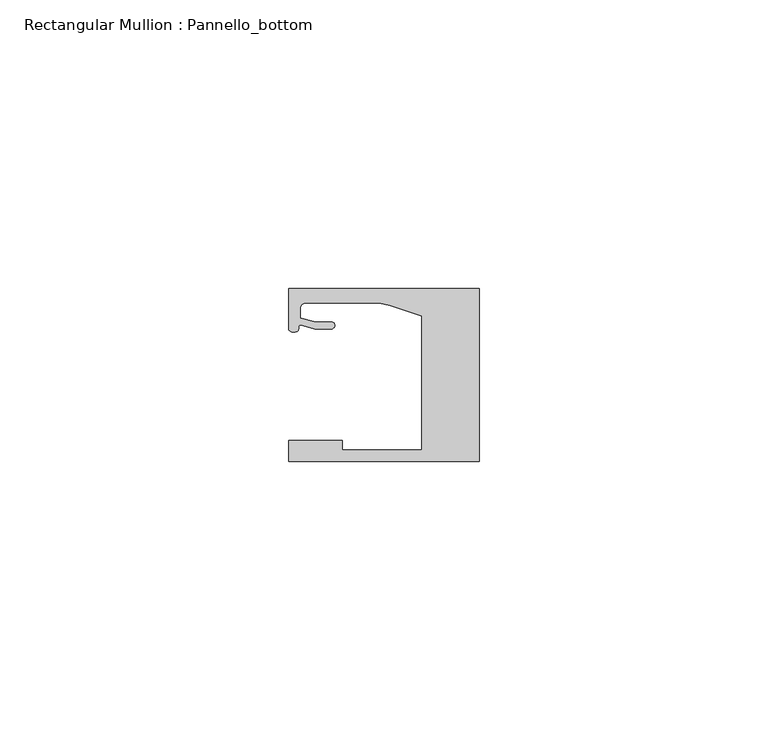
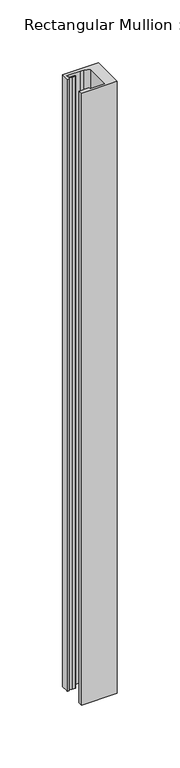
"""IFC4 building model written with IfcOpenShell, lengths in millimetres: member geometry, Rectangular Mullion : Pannello_bottom."""

from ifc_helpers import new_model, si_unit, frame, origin, place, context, project, spatial, polyline, circle_curve, source, transform, mapped, element, save
from ifc_brep_helpers import plane_surface, cylinder_surface, revolved_surface, extruded_surface, spline_curve, advanced_brep


def rectangular_mullion_pannello_bottom_823d01f1(model_context):
    return source(origin(), model_context, "Body", "AdvancedBrep", [
        advanced_brep(
        [(-33.0, -15.0, 0.0), (0.0, -15.0, 0.0), (0.0, 15.0, 0.0), (-33.0000135, 15.0, 0.0), (-33.0000135, 8.0000472, 0.0), (-30.9223017, 8.6490241, 0.0), (-28.4999305, 7.9999523, 0.0), (-25.59998, 7.9999523, 0.0), (-25.59998, 9.1999523, 0.0), (-28.3419477, 9.1999523, 0.0), (-31.0, 9.9121746, 0.0), (-31.0, 11.4999419, 0.0), (-30.0000002, 12.4999419, 0.0), (-18.5493024, 12.4999438, 0.0), (-15.4591336, 12.0105099, 0.0), (-9.9999723, 10.2367227, 0.0), (-9.9999723, -13.0000004, 0.0), (-23.700041, -13.0000004, 0.0), (-23.700041, -11.3000004, 0.0), (-33.0, -11.3000004, 0.0), (-33.0, -15.0, -595.0), (-33.0, -11.3000004, -595.0), (-23.700041, -11.3000004, -595.0), (-23.700041, -13.0000004, -595.0), (-9.9999723, -13.0000004, -595.0), (-9.9999723, 10.2367227, -595.0), (-15.4591336, 12.0105099, -595.0), (-18.5493024, 12.4999438, -595.0), (-30.0000002, 12.4999419, -595.0), (-31.0, 11.4999419, -595.0), (-31.0, 9.9121746, -595.0), (-28.3419477, 9.1999523, -595.0), (-25.59998, 9.1999523, -595.0), (-25.59998, 7.9999523, -595.0), (-28.4999305, 7.9999523, -595.0), (-30.9223017, 8.6490241, -595.0), (-33.0000135, 8.0000472, -595.0), (-33.0000135, 15.0, -595.0), (0.0, 15.0, -595.0), (0.0, -15.0, -595.0)],
        [
            (0, 1),
            (1, 2),
            (2, 3),
            (3, 4),
            (4, 5, spline_curve(3, [(-33.0000135, 8.0000472, 0.0), (-33.0000135, 7.457047519, 0.0), (-32.262327879, 7.456527435, 0.0), (-31.357433266, 7.563996614, 0.0), (-31.305645054, 7.690065204, 0.0), (-31.298563602, 8.366228555, 0.0), (-31.312054066, 8.717747958, 0.0), (-30.9223017, 8.6490241, 0.0)], [4, 2, 2, 4], [0.0, 0.0027053965905959043, 0.0058611956533709, 0.007702013405570312])),
            (5, 6),
            (6, 7),
            (7, 8, circle_curve(frame((-25.59998, 8.5999523, 0.0), z_axis=(0.0, 0.0, 1.0), x_axis=(0.0, 1.0, 0.0)), 0.6)),
            (8, 9),
            (9, 10),
            (10, 11),
            (11, 12, circle_curve(frame((-30.0, 11.4999419, 0.0), z_axis=(0.0, 0.0, -1.0), x_axis=(0.0, 1.0, 0.0)), 1.0)),
            (12, 13),
            (13, 14, circle_curve(frame((-18.5493007, 2.4999438, 0.0), z_axis=(0.0, 0.0, -1.0), x_axis=(0.0, 1.0, 0.0)), 10.0)),
            (14, 15),
            (15, 16),
            (16, 17),
            (17, 18),
            (18, 19),
            (19, 0),
            (20, 21),
            (21, 22),
            (22, 23),
            (23, 24),
            (24, 25),
            (25, 26),
            (26, 27, circle_curve(frame((-18.5493007, 2.4999438, -595.0), z_axis=(0.0, 0.0, 1.0), x_axis=(0.0, 1.0, 0.0)), 10.0)),
            (27, 28),
            (28, 29, circle_curve(frame((-30.0, 11.4999419, -595.0), z_axis=(0.0, 0.0, 1.0), x_axis=(0.0, 1.0, 0.0)), 1.0)),
            (29, 30),
            (30, 31),
            (31, 32),
            (32, 33, circle_curve(frame((-25.59998, 8.5999523, -595.0), z_axis=(0.0, 0.0, -1.0), x_axis=(0.0, 1.0, 0.0)), 0.6)),
            (33, 34),
            (34, 35),
            (35, 36, spline_curve(3, [(-30.9223017, 8.6490241, -595.0), (-31.312054066, 8.717747958, -595.0), (-31.298563602, 8.366228555, -595.0), (-31.305645054, 7.690065204, -595.0), (-31.357433266, 7.563996614, -595.0), (-32.262327879, 7.456527435, -595.0), (-33.0000135, 7.457047519, -595.0), (-33.0000135, 8.0000472, -595.0)], [4, 2, 2, 4], [0.0, 0.001840817752199412, 0.004996616814974408, 0.007702013405570312])),
            (36, 37),
            (37, 38),
            (38, 39),
            (39, 20),
            (0, 20),
            (39, 1),
            (38, 2),
            (37, 3),
            (36, 4),
            (35, 5),
            (34, 6),
            (33, 7),
            (32, 8),
            (31, 9),
            (30, 10),
            (29, 11),
            (28, 12),
            (27, 13),
            (26, 14),
            (25, 15),
            (24, 16),
            (23, 17),
            (22, 18),
            (21, 19),
        ],
        [
            plane_surface(frame((0.0, -36.2491502, 0.0), z_axis=(0.0, 0.0, 1.0), x_axis=(-1.0, 0.0, 0.0))),
            plane_surface(frame((0.0, -36.2491502, -595.0), z_axis=(0.0, 0.0, -1.0), x_axis=(-1.0, 0.0, 0.0))),
            plane_surface(frame((-33.0, -15.0, 0.0), z_axis=(0.0, -1.0, 0.0), x_axis=(0.0, 0.0, -1.0))),
            plane_surface(frame((0.0, -15.0, 0.0), z_axis=(1.0, 0.0, 0.0), x_axis=(0.0, 0.0, -1.0))),
            plane_surface(frame((0.0, 15.0, 0.0), z_axis=(0.0, 1.0, 0.0), x_axis=(0.0, 0.0, -1.0))),
            plane_surface(frame((-33.0000135, 15.0, 0.0), z_axis=(-1.0, 0.0, 0.0), x_axis=(0.0, 0.0, -1.0))),
            extruded_surface(spline_curve(3, [(-33.0000135, 8.0000472, -595.0), (-33.0000135, 7.457047519, -595.0), (-32.262327879, 7.456527435, -595.0), (-31.357433266, 7.563996614, -595.0), (-31.305645054, 7.690065204, -595.0), (-31.298563602, 8.366228555, -595.0), (-31.312054066, 8.717747958, -595.0), (-30.9223017, 8.6490241, -595.0)], [4, 2, 2, 4], [0.0, 0.0027053965905959043, 0.0058611956533709, 0.007702013405570312]), (0.0, 0.0, 595.0), 595.0),
            plane_surface(frame((-30.9223017, 8.6490241, 0.0), z_axis=(-0.25881883200192934, -0.9659258833891746, 0.0), x_axis=(0.0, 0.0, -1.0))),
            plane_surface(frame((-28.4999305, 7.9999523, 0.0), z_axis=(0.0, -1.0, 0.0), x_axis=(0.0, 0.0, -1.0))),
            cylinder_surface(frame((-25.59998, 8.5999523, 0.0), z_axis=(0.0, 0.0, 1.0), x_axis=(0.0, 1.0, 0.0)), 0.6),
            plane_surface(frame((-25.59998, 9.1999523, 0.0), z_axis=(0.0, 1.0, 0.0), x_axis=(0.0, 0.0, -1.0))),
            plane_surface(frame((-28.3419477, 9.1999523, 0.0), z_axis=(0.25881883204288636, 0.9659258833782002, 0.0), x_axis=(0.0, 0.0, -1.0))),
            plane_surface(frame((-31.0, 9.9121746, 0.0), z_axis=(1.0, 0.0, 0.0), x_axis=(0.0, 0.0, -1.0))),
            revolved_surface(polyline([(-30.0, 12.4999419, -595.0), (-30.0, 12.4999419, 0.0)]), (-30.0, 11.4999419, 0.0), (0.0, 0.0, -1.0)),
            plane_surface(frame((-30.0000002, 12.4999419, 0.0), z_axis=(1.6923026533778639e-07, -0.9999999999999858, 0.0), x_axis=(0.0, 0.0, -1.0))),
            revolved_surface(polyline([(-18.5493007, 12.4999438, -595.0), (-18.5493007, 12.4999438, 0.0)]), (-18.5493007, 2.4999438, 0.0), (0.0, 0.0, -1.0)),
            plane_surface(frame((-15.4591336, 12.0105099, 0.0), z_axis=(-0.30901670911956314, -0.9510566089801992, 0.0), x_axis=(0.0, 0.0, -1.0))),
            plane_surface(frame((-9.9999723, 10.2367227, 0.0), z_axis=(-1.0, 0.0, 0.0), x_axis=(0.0, 0.0, -1.0))),
            plane_surface(frame((-9.9999723, -13.0000004, 0.0), z_axis=(0.0, 1.0, 0.0), x_axis=(0.0, 0.0, -1.0))),
            plane_surface(frame((-23.700041, -13.0000004, 0.0), z_axis=(1.0, 0.0, 0.0), x_axis=(0.0, 0.0, -1.0))),
            plane_surface(frame((-23.700041, -11.3000004, 0.0), z_axis=(0.0, 1.0, 0.0), x_axis=(0.0, 0.0, -1.0))),
            plane_surface(frame((-33.0, -11.3000004, 0.0), z_axis=(-1.0, 0.0, 0.0), x_axis=(0.0, 0.0, -1.0))),
        ],
        [
            (0, [[1, 2, 3, 4, 5, 6, 7, 8, 9, 10, 11, 12, 13, 14, 15, 16, 17, 18, 19, 20]]),
            (1, [[21, 22, 23, 24, 25, 26, 27, 28, 29, 30, 31, 32, 33, 34, 35, 36, 37, 38, 39, 40]]),
            (2, [[-1, 41, -40, 42]]),
            (3, [[-2, -42, -39, 43]]),
            (4, [[-3, -43, -38, 44]]),
            (5, [[-4, -44, -37, 45]]),
            (6, [[-5, -45, -36, 46]]),
            (7, [[-6, -46, -35, 47]]),
            (8, [[-7, -47, -34, 48]]),
            (9, [[-8, -48, -33, 49]]),
            (10, [[-9, -49, -32, 50]]),
            (11, [[-10, -50, -31, 51]]),
            (12, [[-11, -51, -30, 52]]),
            (13, [[-12, -52, -29, 53]]),
            (14, [[-13, -53, -28, 54]]),
            (15, [[-14, -54, -27, 55]]),
            (16, [[-15, -55, -26, 56]]),
            (17, [[-16, -56, -25, 57]]),
            (18, [[-17, -57, -24, 58]]),
            (19, [[-18, -58, -23, 59]]),
            (20, [[-19, -59, -22, 60]]),
            (21, [[-20, -60, -21, -41]]),
        ],
    ),
    ])


if __name__ == "__main__":
    model = new_model("IFC4")
    model_context = context("Model", 3, world=origin())
    ifc_project = project(units=[si_unit("LENGTHUNIT", "METRE", prefix="MILLI")], contexts=[model_context])
    site = spatial("IfcSite", under=ifc_project)
    building = spatial("IfcBuilding", under=site)
    placement = place(None, origin())
    rectangular_mullion_pannello_bottom_shape = rectangular_mullion_pannello_bottom_823d01f1(model_context)
    element("IfcMember", 1, ObjectType="Rectangular Mullion : Pannello_bottom", at=placement, inside=building, context=model_context, shape_type="MappedRepresentation", body=[
        mapped(rectangular_mullion_pannello_bottom_shape, transform((0.0, 0.0, 0.0), x_axis=(1.0, 0.0, 0.0), y_axis=(0.0, 1.0, 0.0), z_axis=(0.0, 0.0, 1.0))),
    ])
    save(model, "model.ifc")

# Revit data of these elements
# Type "Rectangular Mullion : Pannello_bottom"
#   built-in parameter 1007322 = 0.0984252 (stored number, unit not read)
#   built-in parameter 1007321 = 0.0328083 (stored number, unit not read)
#   built-in parameter 1007320 = 0 (stored number, unit not read)
